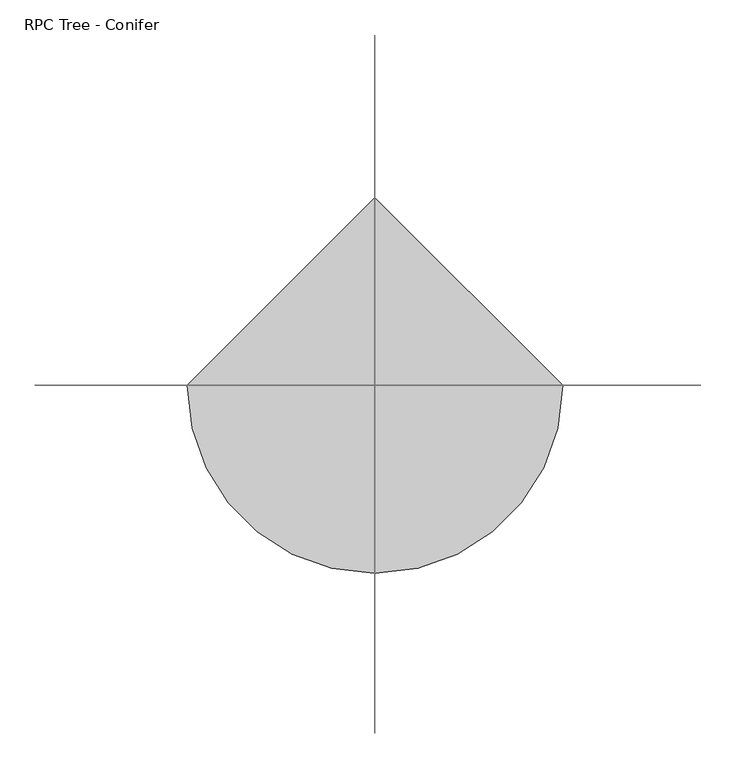
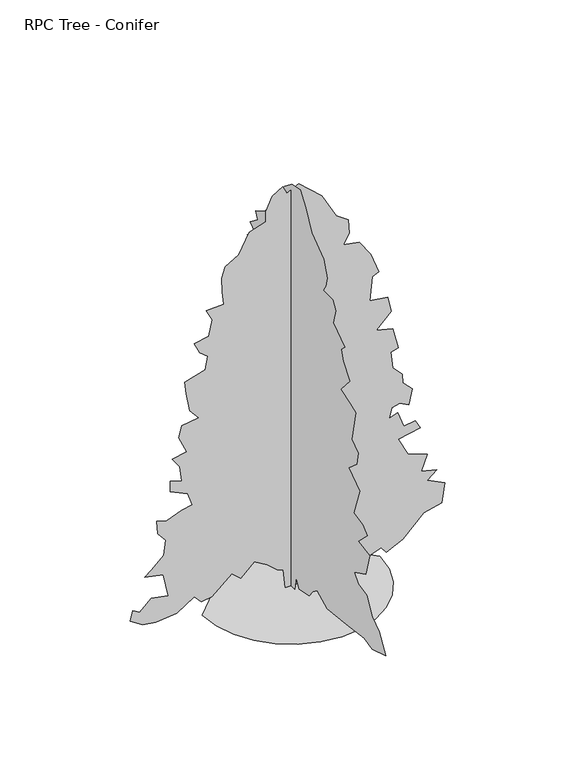
"""IFC4 building model written with IfcOpenShell, lengths in millimetres: geographic element geometry, RPC Tree - Conifer : Colorado Spruce - 4.0 Meters."""

import ifcopenshell
import ifcopenshell.guid

model = None  # the IFC model being written
_history = None  # IfcOwnerHistory: only IFC2X3 demands one
_inside = {}  # id of a spatial element -> (the spatial element, [elements in it])
_under = {}  # id of a project, library or spatial element -> (it, [spatial elements below it])
_declared = {}  # id of a project -> (the project, [libraries it declares])
_typed = {}  # id of a type object -> (the type object, [elements of that type])
_made_of = {}  # id of a material, layer set ... -> (it, [elements and type objects made of it])


def new_model(schema):
    """Start an empty IFC model of exactly this schema.

    Asked for "IFC4X3", IfcOpenShell would pick the latest addendum, in which some entities
    have other attributes; the version numbers below select the first issue.
    IFC2X3 requires an IfcOwnerHistory on every rooted entity: one is made here for all.
    """
    global model, _history
    if schema == "IFC4X3":
        model = ifcopenshell.file(schema_version=(4, 3, 0, 0))
    else:
        model = ifcopenshell.file(schema=schema)
    _inside.clear()
    _under.clear()
    _declared.clear()
    _typed.clear()
    _made_of.clear()
    _history = None
    if model.schema == "IFC2X3":
        org = make("IfcOrganization", Name="unknown")
        user = make(
            "IfcPersonAndOrganization",
            ThePerson=make("IfcPerson", FamilyName="unknown"),
            TheOrganization=org,
        )
        app = make(
            "IfcApplication",
            ApplicationDeveloper=org,
            Version="unknown",
            ApplicationFullName="unknown",
            ApplicationIdentifier="unknown",
        )
        _history = make(
            "IfcOwnerHistory",
            OwningUser=user,
            OwningApplication=app,
            ChangeAction="ADDED",
            CreationDate=0,
        )
    return model


def make(cls, **values):
    """One entity of the class cls with the attributes given. An attribute that is None is left unset."""
    return model.create_entity(
        cls, **{name: value for name, value in values.items() if value is not None}
    )


def rooted(cls, **values):
    """An entity with a GlobalId (a new one), such as an element, a storey or a relation."""
    return make(cls, GlobalId=ifcopenshell.guid.new(), OwnerHistory=_history, **values)


def si_unit(unit_type, name, prefix=None):
    """IfcSIUnit, for example si_unit("LENGTHUNIT", "METRE", prefix="MILLI")."""
    return make("IfcSIUnit", UnitType=unit_type, Prefix=prefix, Name=name)


def assignment(units):
    """IfcUnitAssignment: the units of a project."""
    return None if units is None else make("IfcUnitAssignment", Units=units)


def point(xyz):
    """IfcCartesianPoint."""
    return None if xyz is None else make("IfcCartesianPoint", Coordinates=xyz)


def direction(xyz):
    """IfcDirection."""
    return None if xyz is None else make("IfcDirection", DirectionRatios=xyz)


def frame(location, z_axis=None, x_axis=None):
    """IfcAxis2Placement3D, a coordinate frame: its origin and axes. An axis left out is left unset."""
    return make(
        "IfcAxis2Placement3D",
        Location=point(location),
        Axis=direction(z_axis),
        RefDirection=direction(x_axis),
    )


def origin():
    """The frame at (0, 0, 0) with its axes left unset."""
    return frame((0.0, 0.0, 0.0))


def place(relative_to, where):
    """IfcLocalPlacement: puts the frame where relative to a parent placement (None: the world)."""
    return make(
        "IfcLocalPlacement", PlacementRelTo=relative_to, RelativePlacement=where
    )


def context(
    kind, dimensions, precision=None, world=None, true_north=None, identifier=None
):
    """IfcGeometricRepresentationContext, for example the 3D "Model" context."""
    return make(
        "IfcGeometricRepresentationContext",
        ContextIdentifier=identifier,
        ContextType=kind,
        CoordinateSpaceDimension=dimensions,
        Precision=precision,
        WorldCoordinateSystem=world,
        TrueNorth=true_north,
    )


def project(units=None, contexts=None):
    """IfcProject with its units and contexts."""
    return rooted(
        "IfcProject",
        Name="project",
        RepresentationContexts=contexts,
        UnitsInContext=assignment(units),
    )


def spatial(cls, under=None, at=None, **own):
    """A site, building, storey or space (cls), placed at a placement, below another one or the project."""
    s = rooted(cls, ObjectPlacement=at, **own)
    if under is not None:
        _under.setdefault(under.id(), (under, []))[1].append(s)
    return s


def point_list(points):
    """IfcCartesianPointList2D or 3D."""
    cls = (
        "IfcCartesianPointList2D" if len(points[0]) == 2 else "IfcCartesianPointList3D"
    )
    return make(cls, CoordList=points)


def triangles(points, corners, closed=None, point_numbers=None):
    """IfcTriangulatedFaceSet: each triangle names its three corners, points numbered from 1."""
    return make(
        "IfcTriangulatedFaceSet",
        Coordinates=point_list(points),
        Closed=closed,
        CoordIndex=corners,
        PnIndex=point_numbers,
    )


def shape(context_of_items, identifier, shape_type, items):
    """IfcShapeRepresentation: the items that make up one representation, for example the "Body"."""
    return make(
        "IfcShapeRepresentation",
        ContextOfItems=context_of_items,
        RepresentationIdentifier=identifier,
        RepresentationType=shape_type,
        Items=items,
    )


def source(mapping_origin, context_of_items, identifier, shape_type, items):
    """IfcRepresentationMap: a shape defined once, which mapped items show again and again."""
    return make(
        "IfcRepresentationMap",
        MappingOrigin=mapping_origin,
        MappedRepresentation=shape(context_of_items, identifier, shape_type, items),
    )


def transform(
    local_origin,
    x_axis=None,
    y_axis=None,
    z_axis=None,
    scale=None,
    scale2=None,
    scale3=None,
    uniform=True,
):
    """IfcCartesianTransformationOperator3D, or its non-uniform kind. x_axis, y_axis, z_axis: its Axis1, 2, 3."""
    if uniform:
        return make(
            "IfcCartesianTransformationOperator3D",
            Axis1=direction(x_axis),
            Axis2=direction(y_axis),
            LocalOrigin=point(local_origin),
            Scale=scale,
            Axis3=direction(z_axis),
        )
    return make(
        "IfcCartesianTransformationOperator3DnonUniform",
        Axis1=direction(x_axis),
        Axis2=direction(y_axis),
        LocalOrigin=point(local_origin),
        Scale=scale,
        Axis3=direction(z_axis),
        Scale2=scale2,
        Scale3=scale3,
    )


def mapped(mapping_source, mapping_target):
    """IfcMappedItem: shows the shape of a source again, moved by a transform."""
    return make(
        "IfcMappedItem", MappingSource=mapping_source, MappingTarget=mapping_target
    )


def made_of(thing, what):
    """Note that an element or type object is made of a material, layer set ...; save() writes the relation."""
    if what is not None:
        _made_of.setdefault(what.id(), (what, []))[1].append(thing)
    return thing


def element(
    cls,
    number,
    at=None,
    inside=None,
    cuts=None,
    type_object=None,
    material=None,
    context=None,
    identifier="Body",
    shape_type=None,
    held_by="IfcProductDefinitionShape",
    body=None,
    shapes=None,
    **own,
):
    """One element of the class cls, such as IfcWall. Its Tag is "e" and its number.

    at: its placement. inside: the storey or other place that contains it. cuts: it is an
    opening in that element (IfcRelVoidsElement). A single representation is given by context,
    identifier, shape_type and body (its items); several are given by shapes. held_by: the class
    of the entity that holds the representations. save() writes the other relations.
    """
    e = rooted(cls, Tag="e%d" % number, ObjectPlacement=at, **own)
    if body is not None:
        shapes = [shape(context, identifier, shape_type, body)]
    if shapes is not None:
        e.Representation = make(held_by, Representations=shapes)
    if inside is not None:
        _inside.setdefault(inside.id(), (inside, []))[1].append(e)
    if cuts is not None:
        rooted(
            "IfcRelVoidsElement", RelatingBuildingElement=cuts, RelatedOpeningElement=e
        )
    if type_object is not None:
        _typed.setdefault(type_object.id(), (type_object, []))[1].append(e)
    return made_of(e, material)


def aggregate(whole, parts):
    """IfcRelAggregates: a whole, such as a stair, and the parts it consists of."""
    return rooted("IfcRelAggregates", RelatingObject=whole, RelatedObjects=parts)


def save(model, path):
    """Write the relations noted so far, then the file.

    IfcRelAggregates (storeys below a building ...), IfcRelContainedInSpatialStructure (elements
    in a storey), IfcRelDefinesByType, IfcRelAssociatesMaterial and IfcRelDeclares: one each for
    every whole, place, type object, material and project.
    """
    for whole, parts in _under.values():
        aggregate(whole, parts)
    for where, things in _inside.values():
        rooted(
            "IfcRelContainedInSpatialStructure",
            RelatedElements=things,
            RelatingStructure=where,
        )
    for kind, things in _typed.values():
        rooted("IfcRelDefinesByType", RelatedObjects=things, RelatingType=kind)
    for what, things in _made_of.values():
        rooted("IfcRelAssociatesMaterial", RelatedObjects=things, RelatingMaterial=what)
    for by, libraries in _declared.values():
        rooted("IfcRelDeclares", RelatingContext=by, RelatedDefinitions=libraries)
    model.write(path)


def rpc_tree_conifer_283005fb(model_context):
    return source(origin(), model_context, "Body", "Tessellation", [
        triangles([(0.1966733, 49.8244978, 3.62e-05), (0.1966808, 76.8972503, 209.8139919), (0.1966851, 110.7382534, 304.5674924), (0.1966885, 232.565492, 236.886758), (0.1966934, 381.4650152, 175.9729979), (0.1967001, 550.6699851, 148.90025), (0.1967079, 720.3449844, 156.1022449), (0.1967054, 740.1799656, 40.6092491), (0.1967132, 862.0074858, 121.827502), (0.1967165, 991.2750315, 36.3350005), (0.1967216, 1085.3575155, 67.6820016), (0.1967296, 1268.1000675, 60.913751), (0.1967359, 1356.0849586, 142.1320039), (0.1967499, 1545.5950481, 324.872503), (0.1967463, 1430.5350655, 379.0174902), (0.1967428, 1329.0124832, 412.8600102), (0.1967383, 1234.4449997, 404.9599837), (0.1967407, 1213.9525005, 514.3824835), (0.1967447, 1241.024976, 609.1374919), (0.1967522, 1335.779948, 717.4275026), (0.1967485, 1241.024976, 737.7325132), (0.1967539, 1315.4749374, 805.4150099), (0.1967498, 1200.4174982, 839.2550228), (0.1967461, 1078.589978, 900.169982), (0.1967471, 1015.9549931, 1025.5049915), (0.1967554, 1173.3450228, 1069.3749882), (0.1967602, 1241.024976, 1130.2874765), (0.1967569, 1153.0400122, 1150.5924871), (0.1967529, 1004.1400166, 1238.5800671), (0.1967593, 1112.429991, 1292.7250179), (0.196765, 1121.189994, 1470.9574528), (0.19676, 997.3700083, 1489.0025723), (0.196756, 889.0800339, 1516.0750477), (0.1967604, 905.0550035, 1639.3949913), (0.1967674, 1036.9399767, 1676.5725185), (0.1967726, 1065.0525049, 1807.1074287), (0.1967671, 956.7625305, 1786.8025635), (0.196768, 888.3749897, 1918.5275173), (0.1967741, 963.5299953, 2010.1524479), (0.1967722, 868.7750233, 2091.3700195), (0.1967785, 963.5299953, 2159.0525162), (0.1967813, 990.6024708, 2213.197467), (0.196777, 821.3974646, 2321.4899849), (0.1967781, 801.0925266, 2389.1700108), (0.1967862, 936.4575199, 2456.8523621), (0.1967861, 875.5424881, 2544.8498978), (0.1967818, 740.1799656, 2605.7499596), (0.1967888, 828.1650021, 2707.2748672), (0.1967872, 733.41003, 2795.2500206), (0.1967844, 611.5849806, 2883.2498817), (0.1967873, 604.8150086, 2991.5499573), (0.1967932, 706.3374819, 3038.9249725), (0.1967915, 631.8899912, 3093.074865), (0.1967882, 543.9024839, 3113.3750793), (0.1967957, 658.9624666, 3194.5750648), (0.1967931, 537.1349828, 3289.3500938), (0.1967966, 570.9749957, 3357.0250328), (0.1967927, 428.8425013, 3438.2500168), (0.1967912, 313.7824822, 3560.0751389), (0.1967925, 237.8634971, 3716.3499023), (0.1967912, 97.2017522, 3884.9500763), (0.196789, -11.0894496, 3972.924939), (0.1967837, -146.4532518, 4000.0000305), (0.1967759, -241.2080059, 3878.1749084), (0.196766, -335.9624874, 3688.6751381), (0.196753, -532.2400054, 3546.5250938), (0.1967459, -586.3849926, 3390.8750015), (0.1967443, -559.3125172, 3296.0999725), (0.196744, -525.4725042, 3235.1999107), (0.1967374, -674.3724998, 3235.1999107), (0.1967328, -721.7499859, 3153.9749268), (0.1967304, -681.1399647, 3011.849881), (0.1967181, -870.6499815, 2883.2498817), (0.1967192, -809.7350224, 2829.0999893), (0.1967147, -843.5775061, 2727.5750816), (0.196706, -951.8674805, 2598.9750824), (0.1967076, -802.9674849, 2429.780032), (0.1966991, -959.7425085, 2380.804969), (0.1966941, -1046.6225252, 2341.7949955), (0.1966879, -985.7074934, 2043.9925335), (0.1966812, -1087.2324738, 1969.542572), (0.1966785, -1066.9275358, 1847.7149792), (0.1966808, -938.3300074, 1732.6574673), (0.1966693, -1114.3050219, 1610.8300198), (0.1966655, -1012.7825123, 1333.3325684), (0.1966581, -1161.6825079, 1306.2599476), (0.1966529, -1236.132542, 1245.3475319), (0.1966552, -1087.2324738, 1096.4475363), (0.1966459, -1276.7399471, 1069.3749882), (0.1966422, -1209.0599939, 846.0224876), (0.1966478, -1026.3175146, 758.0375238), (0.1966426, -1087.2324738, 676.8200249), (0.1966355, -1229.3624611, 649.7474768), (0.1966269, -1317.3499683, 494.0775092), (0.1966194, -1432.409951, 412.8600102), (0.1966096, -1533.9325333, 236.886758), (0.1966172, -1317.3499683, 169.2047519), (0.1966241, -1184.517524, 199.5652534), (0.1966359, -895.4949766, 164.0745054), (0.1966487, -586.3849926, 128.5955028), (0.1966584, -423.9474875, 209.8139919), (0.1966598, -356.267498, 155.6682416), (0.1966603, -295.3525025, 81.2182529), (0.1966665, -132.9167506, 47.3774997), (0.1966712, -85.8942484, 133.3167535), (0.1966685, -58.4667483, 3.3e-05), (-51.204578, 1.3e-06, 3.62e-05), (-71.5090799, -2.08e-05, 182.7412439), (-125.6545758, -2.01e-05, 203.0457458), (-220.4093299, -2.09e-05, 284.2650071), (-342.2358327, -2.06e-05, 358.7149867), (-470.8333248, 3.2e-06, 236.886758), (-552.0508238, 2.3e-06, 311.3375007), (-741.5608406, 1.52e-05, 148.90025), (-836.7233459, 1.86e-05, 136.9905027), (-903.9958385, 1.73e-05, 209.8139919), (-1066.4333799, 2.7e-05, 101.5230001), (-1262.7108616, 4.83e-05, 81.2184982), (-1384.5383091, 5.1e-05, 101.5230001), (-1499.5982918, 5.11e-05, 175.9729979), (-1479.2934265, 4.63e-05, 270.7274976), (-1411.6107845, 4.61e-05, 230.1184938), (-1303.318412, 2.38e-05, 331.6425113), (-1147.6508789, 2.04e-05, 304.5674924), (-1193.5583239, 1.17e-05, 528.1124957), (-1364.2332985, 1.53e-05, 561.7600059), (-1303.318412, 1.14e-05, 609.1374919), (-1188.2608274, 3.1e-06, 717.4275026), (-1167.9558895, -3.8e-06, 859.5600334), (-1242.405851, -5.5e-06, 947.547468), (-1255.9433968, -1.09e-05, 1076.1425257), (-1161.188352, -1.25e-05, 1049.0699776), (-1019.0558212, -3.37e-05, 1103.2150011), (-924.3008492, -3.74e-05, 1123.5200117), (-964.9108704, -4.17e-05, 1245.3475319), (-1127.4908449, -4.02e-05, 1321.492448), (-1127.3458683, -4.5e-05, 1428.0875404), (-1019.0558212, -4.67e-05, 1394.2474548), (-1037.3183693, -5.26e-05, 1538.1075691), (-1107.0433285, -5.5e-05, 1637.9024952), (-971.6783352, -6.02e-05, 1664.9749706), (-1046.1283693, -6.53e-05, 1827.4099686), (-1019.0558212, -7.09e-05, 1935.7024864), (-863.3883608, -9.13e-05, 1962.7749619), (-944.6058598, -9.31e-05, 2057.5299339), (-978.4458727, -0.0001002, 2240.2699425), (-991.9833458, -0.000105, 2355.3300705), (-802.473329, -0.0001134, 2416.2424862), (-775.4008535, -0.0001196, 2538.0750206), (-849.8508877, -0.0001201, 2598.9750824), (-903.9958385, -0.0001233, 2707.2748672), (-766.3633238, -0.000143, 2730.4499062), (-734.7908323, -0.0001508, 2883.2498817), (-788.9358559, -0.000154, 2991.5499573), (-626.5008579, -0.0001591, 2998.3001266), (-640.0358603, -0.0001645, 3126.9001259), (-646.8058685, -0.0001703, 3262.2750023), (-612.9633848, -0.0001759, 3363.79991), (-487.5108315, -0.0001976, 3440.9251442), (-389.6133187, -0.0002089, 3627.7500778), (-233.9455858, -0.0002156, 3675.1250931), (-233.9455858, -0.0002202, 3776.6500008), (-173.0318439, -0.0002277, 3905.25), (-78.277326, -0.0002333, 3966.1500618), (-37.6680791, -0.0002312, 3891.699955), (70.622924, -0.0002513, 3945.8501381), (287.2041627, -0.000249, 3749.5749092), (422.5691923, -0.0002276, 3505.9249557), (537.629175, -0.0002419, 3424.6999718), (544.3966762, -0.0002216, 3289.3500938), (490.251689, -0.0002157, 3194.5750648), (639.1516119, -0.000219, 3167.5249718), (747.441659, -0.0002152, 3011.849881), (821.8916204, -0.0002087, 2815.5749428), (760.3216141, -0.0002054, 2783.5498627), (733.9066566, -0.0001945, 2558.3749443), (903.1091194, -0.0001984, 2531.3001434), (936.9516758, -0.0001927, 2382.4025459), (794.819145, -0.0001824, 2247.0400234), (950.4866781, -0.0001853, 2206.4300022), (1004.6341724, -0.000163, 1996.6150475), (930.1816675, -0.0001602, 1983.0799725), (950.4866781, -0.0001535, 1820.6425037), (1039.9941507, -0.0001518, 1722.8699833), (1045.2416502, -0.0001482, 1637.9024952), (1133.2291574, -0.0001468, 1549.9149879), (1099.3866737, -0.0001392, 1401.015065), (1018.1691748, -0.0001389, 1448.392551), (943.7191406, -0.0001358, 1428.0875404), (916.6466652, -0.0001307, 1333.3325684), (997.8641642, -0.0001343, 1360.4050438), (1052.009115, -0.000129, 1204.7375107), (1160.3016329, -0.0001331, 1225.0425213), (1207.6791189, -0.0001306, 1137.055014), (1004.6341724, -0.0001227, 1096.4475363), (1092.6191362, -0.000103, 920.4725218), (1275.3616882, -0.0001199, 852.7924959), (1216.884153, -9.7e-05, 703.8949711), (1363.3465794, -9.98e-05, 670.0500166), (1275.3616882, -9.39e-05, 595.5999825), (1437.7966862, -9.51e-05, 514.3824835), (1410.7242107, -8.58e-05, 324.872503), (1241.5191319, -7.9e-05, 284.2650071), (1046.1716806, -6.47e-05, 94.2452466), (889.5741171, -4.22e-05, 20.3044996), (842.1966311, -4.35e-05, 81.2182529), (664.5366177, -3.55e-05, 20.9521254), (476.7141795, -2.96e-05, 13.5363501), (402.2641817, -3.04e-05, 81.2182529), (233.0594117, -2.8e-05, 142.1320039), (73.3656708, -2.18e-05, 109.4187482), (57.0864228, -1.64e-05, 3.3e-05), (-828.2308411, -4.6e-06, 5.94e-05), (-806.3283262, -189.8204993, 5.31e-05), (-743.9558252, -364.1399826, 4.6e-05), (-646.1033678, -517.9650046, 3.85e-05), (-517.7683233, -646.3000128, 3.09e-05), (-363.9433013, -744.1524702, 2.34e-05), (-189.6238362, -806.5249712, 1.63e-05), (0.1967073, -828.427486, 1e-05), (190.0171625, -806.5249712, 5e-06), (364.3366639, -744.1524702, 1.7e-06), (518.1616859, -646.3000128, 0.0), (646.4966578, -517.9650046, 0.0), (744.3491152, -364.1399826, 1.7e-06), (806.7216162, -189.8204993, 5e-06), (828.624131, 7.68e-05, 1e-05), (0.1965624, 828.427486, 5.94e-05)], [[26, 27, 28], [21, 22, 23], [19, 20, 21], [51, 52, 53], [7, 8, 9], [35, 36, 37], [13, 14, 15], [34, 35, 37], [54, 55, 56], [72, 73, 74], [95, 96, 97], [88, 89, 90], [44, 45, 46], [86, 87, 88], [85, 86, 88], [51, 53, 54], [44, 46, 47], [88, 90, 91], [13, 15, 16], [13, 16, 17], [38, 39, 40], [25, 26, 28], [25, 28, 29], [47, 48, 49], [56, 57, 58], [30, 31, 32], [29, 30, 32], [41, 42, 43], [40, 41, 43], [106, 1, 2], [105, 106, 2], [75, 76, 77], [94, 95, 97], [94, 97, 98], [78, 79, 80], [83, 84, 85], [29, 32, 33], [103, 104, 105], [12, 13, 17], [11, 12, 17], [77, 78, 80], [102, 103, 105], [62, 63, 64], [80, 81, 82], [80, 82, 83], [61, 62, 64], [61, 64, 65], [60, 61, 65], [59, 60, 65], [69, 70, 71], [69, 71, 72], [94, 98, 99], [93, 94, 99], [92, 93, 99], [92, 99, 100], [91, 92, 100], [91, 100, 101], [47, 49, 50], [9, 10, 11], [9, 11, 17], [9, 17, 18], [7, 9, 18], [59, 65, 66], [59, 66, 67], [59, 67, 68], [59, 68, 69], [58, 59, 69], [56, 58, 69], [54, 56, 69], [54, 69, 72], [51, 54, 72], [50, 51, 72], [50, 72, 74], [50, 74, 75], [50, 75, 77], [47, 50, 77], [44, 47, 77], [43, 44, 77], [40, 43, 77], [40, 77, 80], [40, 80, 83], [38, 40, 83], [38, 83, 85], [37, 38, 85], [34, 37, 85], [33, 34, 85], [29, 33, 85], [25, 29, 85], [25, 85, 88], [25, 88, 91], [25, 91, 101], [25, 101, 102], [24, 25, 102], [23, 24, 102], [21, 23, 102], [105, 2, 3], [102, 105, 3], [21, 102, 3], [21, 3, 4], [21, 4, 5], [21, 5, 6], [21, 6, 7], [21, 7, 18], [19, 21, 18], [125, 126, 127], [198, 199, 200], [153, 154, 155], [139, 140, 141], [130, 131, 132], [120, 121, 122], [119, 120, 122], [186, 187, 188], [136, 137, 138], [135, 136, 138], [150, 151, 152], [193, 194, 195], [192, 193, 195], [125, 127, 128], [180, 181, 182], [163, 164, 165], [185, 186, 188], [196, 197, 198], [190, 191, 192], [111, 112, 113], [212, 107, 108], [211, 212, 108], [173, 174, 175], [149, 150, 152], [179, 180, 182], [129, 130, 132], [146, 147, 148], [204, 205, 206], [200, 201, 202], [200, 202, 203], [162, 163, 165], [190, 192, 195], [165, 166, 167], [118, 119, 122], [118, 122, 123], [118, 123, 124], [117, 118, 124], [116, 117, 124], [176, 177, 178], [176, 178, 179], [129, 132, 133], [185, 188, 189], [142, 143, 144], [141, 142, 144], [161, 162, 165], [161, 165, 167], [161, 167, 168], [116, 124, 125], [145, 146, 148], [144, 145, 148], [114, 115, 116], [113, 114, 116], [113, 116, 125], [113, 125, 128], [113, 128, 129], [113, 129, 133], [113, 133, 134], [111, 113, 134], [168, 169, 170], [168, 170, 171], [161, 168, 171], [160, 161, 171], [159, 160, 171], [158, 159, 171], [157, 158, 171], [156, 157, 171], [155, 156, 171], [171, 172, 173], [171, 173, 175], [155, 171, 175], [155, 175, 176], [153, 155, 176], [152, 153, 176], [149, 152, 176], [149, 176, 179], [148, 149, 179], [144, 148, 179], [144, 179, 182], [144, 182, 183], [141, 144, 183], [139, 141, 183], [138, 139, 183], [135, 138, 183], [134, 135, 183], [111, 134, 183], [110, 111, 183], [110, 183, 184], [110, 184, 185], [110, 185, 189], [110, 189, 190], [110, 190, 195], [109, 110, 195], [108, 109, 195], [211, 108, 195], [210, 211, 195], [210, 195, 196], [209, 210, 196], [209, 196, 198], [208, 209, 198], [207, 208, 198], [206, 207, 198], [204, 206, 198], [203, 204, 198], [200, 203, 198], [227, 228, 213], [226, 227, 213], [226, 213, 214], [225, 226, 214], [225, 214, 215], [225, 215, 216], [224, 225, 216], [223, 224, 216], [223, 216, 217], [223, 217, 218], [223, 218, 219], [223, 219, 220], [223, 220, 221], [223, 221, 222]], closed=False),
    ])


if __name__ == "__main__":
    model = new_model("IFC4")
    model_context = context("Model", 3, world=origin())
    ifc_project = project(units=[si_unit("LENGTHUNIT", "METRE", prefix="MILLI")], contexts=[model_context])
    site = spatial("IfcSite", under=ifc_project)
    building = spatial("IfcBuilding", under=site)
    placement = place(None, origin())
    rpc_tree_conifer_shape = rpc_tree_conifer_283005fb(model_context)
    element("IfcGeographicElement", 1, ObjectType="RPC Tree - Conifer : Colorado Spruce - 4.0 Meters", at=placement, inside=building, context=model_context, shape_type="MappedRepresentation", body=[
        mapped(rpc_tree_conifer_shape, transform((0.0, 0.0, 0.0), x_axis=(1.0, 0.0, 0.0), y_axis=(0.0, 1.0, 0.0), z_axis=(0.0, 0.0, 1.0))),
    ])
    save(model, "model.ifc")

# Revit data of these elements
# Type "RPC Tree - Conifer : Colorado Spruce - 4.0 Meters"
#   built-in parameter 1005198 = "{2, 15},{39, RPC-16-G0M4-N9PX-U6TN-C000-ST1L-LVER-AU},{1, 0},{1, 0},{2, 13},{1, 8},{5, Color},{1, 0},{1, 0},{3, 0.8},{3, 0.8},{3, 0.8},{1, 8},{7, BBoxMin},{1, 0},{1, 0},{1, 0},{1, 0},{1, 0},{1, 8},{7, BBoxMax},{1, 0},{1, 0},{1, 0},{1, 0},{1, 0},{2, 11},{9, RPCTypeId},{1, 0},{1, 0},{39, RPC-16-G0M4-N9PX-U6TN-C000-ST1L-LVER-AU},{1, 6},{14, RPCPlantHeight},{1, 0},{1, 0},{7, 13.1234},{2, 11},{7, keyword},{1, 0},{1, 0},{34, :RPCs:Trees [General]:Geometry:RPC},{2, 11},{8, category},{1, 0},{1, 0},{15, Trees [General]},{2, 11},{12, LocalizedUID},{1, 0},{1, 0},{15, Colorado Spruce},{2, 14},{6, Height},{1, 0},{1, 0},{7, 13.1234},{1, 2},{16, Cast Reflections},{1, 0},{1, 0},{1, 0},{1, 2},{12, Cast Shadows},{1, 0},{1, 0},{1, 1},{1, 2},{9, Lock View},{1, 0},{1, 0},{1, 0},{1, 4},{5, ViewC},{1, 0},{1, 0},{1, 0},{21, assetlibrary_base.fbx},{1, 5},"
#   built-in parameter 1005195 = "RPC-16-G0M4-N9PX-U6TN-C000-ST1L-LVER-AU"
#   Type Comments = "Colorado Spruce"
#   Height = 4000 mm
#   Description = (empty or 0)
#   Default Elevation = 0
